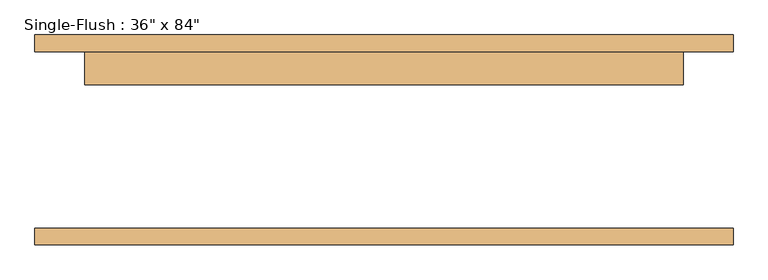
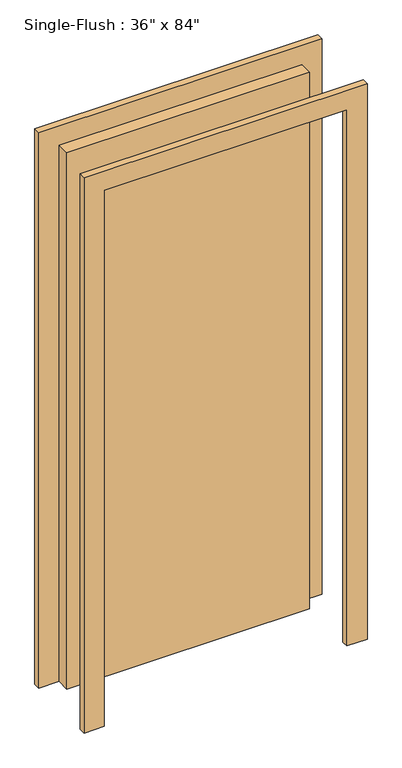
"""IFC4 building model written with IfcOpenShell, lengths in millimetres: door geometry."""

import ifcopenshell
import ifcopenshell.guid

model = None  # the IFC model being written
_history = None  # IfcOwnerHistory: only IFC2X3 demands one
_inside = {}  # id of a spatial element -> (the spatial element, [elements in it])
_under = {}  # id of a project, library or spatial element -> (it, [spatial elements below it])
_declared = {}  # id of a project -> (the project, [libraries it declares])
_typed = {}  # id of a type object -> (the type object, [elements of that type])
_made_of = {}  # id of a material, layer set ... -> (it, [elements and type objects made of it])


def new_model(schema):
    """Start an empty IFC model of exactly this schema.

    Asked for "IFC4X3", IfcOpenShell would pick the latest addendum, in which some entities
    have other attributes; the version numbers below select the first issue.
    IFC2X3 requires an IfcOwnerHistory on every rooted entity: one is made here for all.
    """
    global model, _history
    if schema == "IFC4X3":
        model = ifcopenshell.file(schema_version=(4, 3, 0, 0))
    else:
        model = ifcopenshell.file(schema=schema)
    _inside.clear()
    _under.clear()
    _declared.clear()
    _typed.clear()
    _made_of.clear()
    _history = None
    if model.schema == "IFC2X3":
        org = make("IfcOrganization", Name="unknown")
        user = make(
            "IfcPersonAndOrganization",
            ThePerson=make("IfcPerson", FamilyName="unknown"),
            TheOrganization=org,
        )
        app = make(
            "IfcApplication",
            ApplicationDeveloper=org,
            Version="unknown",
            ApplicationFullName="unknown",
            ApplicationIdentifier="unknown",
        )
        _history = make(
            "IfcOwnerHistory",
            OwningUser=user,
            OwningApplication=app,
            ChangeAction="ADDED",
            CreationDate=0,
        )
    return model


def make(cls, **values):
    """One entity of the class cls with the attributes given. An attribute that is None is left unset."""
    return model.create_entity(
        cls, **{name: value for name, value in values.items() if value is not None}
    )


def rooted(cls, **values):
    """An entity with a GlobalId (a new one), such as an element, a storey or a relation."""
    return make(cls, GlobalId=ifcopenshell.guid.new(), OwnerHistory=_history, **values)


def si_unit(unit_type, name, prefix=None):
    """IfcSIUnit, for example si_unit("LENGTHUNIT", "METRE", prefix="MILLI")."""
    return make("IfcSIUnit", UnitType=unit_type, Prefix=prefix, Name=name)


def assignment(units):
    """IfcUnitAssignment: the units of a project."""
    return None if units is None else make("IfcUnitAssignment", Units=units)


def point(xyz):
    """IfcCartesianPoint."""
    return None if xyz is None else make("IfcCartesianPoint", Coordinates=xyz)


def direction(xyz):
    """IfcDirection."""
    return None if xyz is None else make("IfcDirection", DirectionRatios=xyz)


def frame(location, z_axis=None, x_axis=None):
    """IfcAxis2Placement3D, a coordinate frame: its origin and axes. An axis left out is left unset."""
    return make(
        "IfcAxis2Placement3D",
        Location=point(location),
        Axis=direction(z_axis),
        RefDirection=direction(x_axis),
    )


def origin():
    """The frame at (0, 0, 0) with its axes left unset."""
    return frame((0.0, 0.0, 0.0))


def origin_with_axes():
    """The frame at (0, 0, 0) with the z axis (0, 0, 1) and the x axis (1, 0, 0) written out."""
    return frame((0.0, 0.0, 0.0), z_axis=(0.0, 0.0, 1.0), x_axis=(1.0, 0.0, 0.0))


def place(relative_to, where):
    """IfcLocalPlacement: puts the frame where relative to a parent placement (None: the world)."""
    return make(
        "IfcLocalPlacement", PlacementRelTo=relative_to, RelativePlacement=where
    )


def context(
    kind, dimensions, precision=None, world=None, true_north=None, identifier=None
):
    """IfcGeometricRepresentationContext, for example the 3D "Model" context."""
    return make(
        "IfcGeometricRepresentationContext",
        ContextIdentifier=identifier,
        ContextType=kind,
        CoordinateSpaceDimension=dimensions,
        Precision=precision,
        WorldCoordinateSystem=world,
        TrueNorth=true_north,
    )


def project(units=None, contexts=None):
    """IfcProject with its units and contexts."""
    return rooted(
        "IfcProject",
        Name="project",
        RepresentationContexts=contexts,
        UnitsInContext=assignment(units),
    )


def spatial(cls, under=None, at=None, **own):
    """A site, building, storey or space (cls), placed at a placement, below another one or the project."""
    s = rooted(cls, ObjectPlacement=at, **own)
    if under is not None:
        _under.setdefault(under.id(), (under, []))[1].append(s)
    return s


def polyline(points):
    """IfcPolyline through the points."""
    return make("IfcPolyline", Points=[point(p) for p in points])


def outline(outer, holes=None, kind="AREA"):
    """IfcArbitraryClosedProfileDef: a profile drawn as a closed curve; with holes, ...WithVoids."""
    if holes is None:
        return make("IfcArbitraryClosedProfileDef", ProfileType=kind, OuterCurve=outer)
    return make(
        "IfcArbitraryProfileDefWithVoids",
        ProfileType=kind,
        OuterCurve=outer,
        InnerCurves=holes,
    )


def extrude(swept, where, along, depth):
    """IfcExtrudedAreaSolid: the profile swept, set in the frame where, extruded along a direction by depth."""
    return make(
        "IfcExtrudedAreaSolid",
        SweptArea=swept,
        Position=where,
        ExtrudedDirection=direction(along),
        Depth=depth,
    )


def shape(context_of_items, identifier, shape_type, items):
    """IfcShapeRepresentation: the items that make up one representation, for example the "Body"."""
    return make(
        "IfcShapeRepresentation",
        ContextOfItems=context_of_items,
        RepresentationIdentifier=identifier,
        RepresentationType=shape_type,
        Items=items,
    )


def source(mapping_origin, context_of_items, identifier, shape_type, items):
    """IfcRepresentationMap: a shape defined once, which mapped items show again and again."""
    return make(
        "IfcRepresentationMap",
        MappingOrigin=mapping_origin,
        MappedRepresentation=shape(context_of_items, identifier, shape_type, items),
    )


def transform(
    local_origin,
    x_axis=None,
    y_axis=None,
    z_axis=None,
    scale=None,
    scale2=None,
    scale3=None,
    uniform=True,
):
    """IfcCartesianTransformationOperator3D, or its non-uniform kind. x_axis, y_axis, z_axis: its Axis1, 2, 3."""
    if uniform:
        return make(
            "IfcCartesianTransformationOperator3D",
            Axis1=direction(x_axis),
            Axis2=direction(y_axis),
            LocalOrigin=point(local_origin),
            Scale=scale,
            Axis3=direction(z_axis),
        )
    return make(
        "IfcCartesianTransformationOperator3DnonUniform",
        Axis1=direction(x_axis),
        Axis2=direction(y_axis),
        LocalOrigin=point(local_origin),
        Scale=scale,
        Axis3=direction(z_axis),
        Scale2=scale2,
        Scale3=scale3,
    )


def mapped(mapping_source, mapping_target):
    """IfcMappedItem: shows the shape of a source again, moved by a transform."""
    return make(
        "IfcMappedItem", MappingSource=mapping_source, MappingTarget=mapping_target
    )


def made_of(thing, what):
    """Note that an element or type object is made of a material, layer set ...; save() writes the relation."""
    if what is not None:
        _made_of.setdefault(what.id(), (what, []))[1].append(thing)
    return thing


def element(
    cls,
    number,
    at=None,
    inside=None,
    cuts=None,
    type_object=None,
    material=None,
    context=None,
    identifier="Body",
    shape_type=None,
    held_by="IfcProductDefinitionShape",
    body=None,
    shapes=None,
    **own,
):
    """One element of the class cls, such as IfcWall. Its Tag is "e" and its number.

    at: its placement. inside: the storey or other place that contains it. cuts: it is an
    opening in that element (IfcRelVoidsElement). A single representation is given by context,
    identifier, shape_type and body (its items); several are given by shapes. held_by: the class
    of the entity that holds the representations. save() writes the other relations.
    """
    e = rooted(cls, Tag="e%d" % number, ObjectPlacement=at, **own)
    if body is not None:
        shapes = [shape(context, identifier, shape_type, body)]
    if shapes is not None:
        e.Representation = make(held_by, Representations=shapes)
    if inside is not None:
        _inside.setdefault(inside.id(), (inside, []))[1].append(e)
    if cuts is not None:
        rooted(
            "IfcRelVoidsElement", RelatingBuildingElement=cuts, RelatedOpeningElement=e
        )
    if type_object is not None:
        _typed.setdefault(type_object.id(), (type_object, []))[1].append(e)
    return made_of(e, material)


def aggregate(whole, parts):
    """IfcRelAggregates: a whole, such as a stair, and the parts it consists of."""
    return rooted("IfcRelAggregates", RelatingObject=whole, RelatedObjects=parts)


def save(model, path):
    """Write the relations noted so far, then the file.

    IfcRelAggregates (storeys below a building ...), IfcRelContainedInSpatialStructure (elements
    in a storey), IfcRelDefinesByType, IfcRelAssociatesMaterial and IfcRelDeclares: one each for
    every whole, place, type object, material and project.
    """
    for whole, parts in _under.values():
        aggregate(whole, parts)
    for where, things in _inside.values():
        rooted(
            "IfcRelContainedInSpatialStructure",
            RelatedElements=things,
            RelatingStructure=where,
        )
    for kind, things in _typed.values():
        rooted("IfcRelDefinesByType", RelatedObjects=things, RelatingType=kind)
    for what, things in _made_of.values():
        rooted("IfcRelAssociatesMaterial", RelatedObjects=things, RelatingMaterial=what)
    for by, libraries in _declared.values():
        rooted("IfcRelDeclares", RelatingContext=by, RelatedDefinitions=libraries)
    model.write(path)


def door_e3ca8ffb(model_context):
    return source(origin(), model_context, "Body", "SweptSolid", [
        extrude(outline(polyline([(2209.8, -533.4), (0.0, -533.4), (0.0, -457.2), (2133.6, -457.2), (2133.6, 457.2), (0.0, 457.2), (0.0, 533.4), (2209.8, 533.4), (2209.8, -533.4)])), frame((0.0, 134.9375, 0.0), z_axis=(0.0, 1.0, 0.0), x_axis=(0.0, 0.0, 1.0)), (0.0, 0.0, 1.0), 25.4),
        extrude(outline(polyline([(2209.8, 533.4), (2209.8, -533.4), (0.0, -533.4), (0.0, -457.2), (2133.6, -457.2), (2133.6, 457.2), (0.0, 457.2), (0.0, 533.4), (2209.8, 533.4)])), frame((0.0, -160.3375, 0.0), z_axis=(0.0, 1.0, 0.0), x_axis=(0.0, 0.0, 1.0)), (0.0, 0.0, 1.0), 25.4),
        extrude(outline(polyline([(457.2, 84.1375), (-457.2, 84.1375), (-457.2, 134.9375), (457.2, 134.9375), (457.2, 84.1375)])), origin_with_axes(), (0.0, 0.0, 1.0), 2133.6),
    ])


if __name__ == "__main__":
    model = new_model("IFC4")
    model_context = context("Model", 3, world=origin())
    ifc_project = project(units=[si_unit("LENGTHUNIT", "METRE", prefix="MILLI")], contexts=[model_context])
    site = spatial("IfcSite", under=ifc_project)
    building = spatial("IfcBuilding", under=site)
    placement = place(None, origin())
    door_shape = door_e3ca8ffb(model_context)
    element("IfcDoor", 1, ObjectType="Single-Flush : 36\" x 84\"", at=placement, inside=building, context=model_context, shape_type="MappedRepresentation", body=[
        mapped(door_shape, transform((0.0, 0.0, 0.0), x_axis=(1.0, 0.0, 0.0), y_axis=(0.0, 1.0, 0.0), z_axis=(0.0, 0.0, 1.0))),
    ])
    save(model, "model.ifc")

# Revit data of these elements
# Type "Single-Flush : 36\" x 84\""
#   Type Mark = "1"
#   Assembly Code = "C1020"
#   Thickness = 0' - 2"
#   Height = 7' - 0"
#   Trim Projection Ext = 0' - 1"
#   Trim Projection Int = 0' - 1"
#   Trim Width = 0' - 3"
#   Width = 3' - 0"
#   Door Material = PAINTED STEEL C CHANNEL
#   Frame Material = PAINTED STEEL C CHANNEL
#   Function = (empty or 0)
#   Wall Closure = (empty or 0)
# Element 1 (IfcDoor, "Single-Flush : 36\" x 84\"")
#   Materials on its faces: "PAINTED STEEL C CHANNEL"
# Materials
#   "PAINTED STEEL C CHANNEL": class "Generic", colour RGB 88 62 61, transparency 0, Cost = 0
